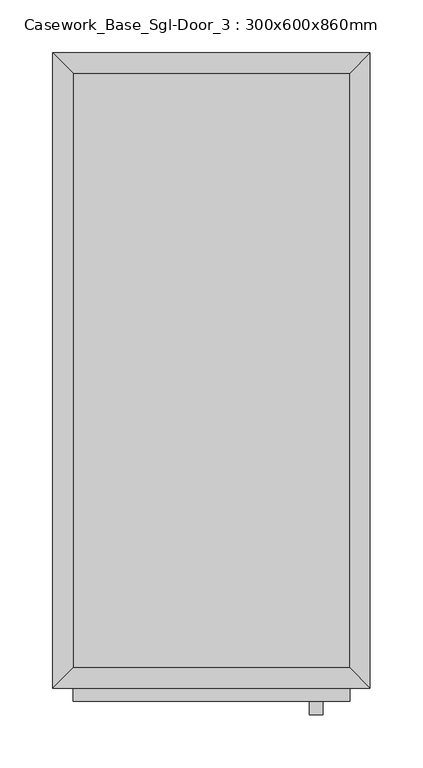
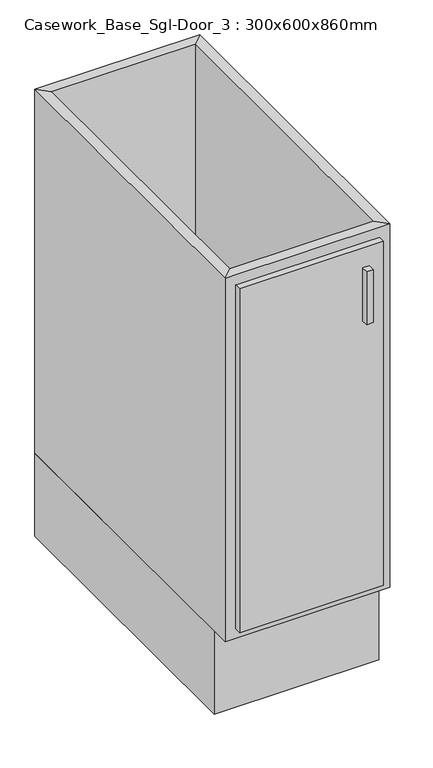
"""IFC4 building model written with IfcOpenShell, lengths in millimetres: furniture geometry, Casework_Base_Sgl-Door_3 : 300x600x860mm."""

from ifc_helpers import new_model, si_unit, frame, origin, origin_with_axes, place, context, project, spatial, polyline, outline, extrude, faceted_brep, source, transform, mapped, element, save


def casework_base_sgl_door_3_300x600x860mm_ce4f0042(model_context):
    return source(origin(), model_context, "Body", "SolidModel", [
        extrude(outline(polyline([(149.6877049, -19.05), (149.6877049, -580.95), (-112.2122951, -580.95), (-112.2122951, -19.05), (149.6877049, -19.05)])), frame((0.0, 0.0, 160.0), z_axis=(0.0, 0.0, 1.0), x_axis=(1.0, 0.0, 0.0)), (0.0, 0.0, 1.0), 19.05),
        faceted_brep([(149.6877049, -580.95, 860.0), (149.6877049, -580.95, 160.0), (-112.2122951, -580.95, 160.0), (-112.2122951, -580.95, 860.0), (168.7377049, -600.0, 860.0), (-131.2622951, -600.0, 860.0), (168.7377049, -600.0, 160.0), (-131.2622951, -600.0, 160.0), (-112.2122951, -19.05, 160.0), (-112.2122951, -19.05, 860.0), (-131.2622951, 0.0, 860.0), (-131.2622951, 0.0, 160.0), (149.6877049, -19.05, 160.0), (149.6877049, -19.05, 860.0), (168.7377049, 0.0, 860.0), (168.7377049, 0.0, 160.0)], [[[0, 1, 2, 3]], [[4, 0, 3, 5]], [[6, 4, 5, 7]], [[1, 6, 7, 2]], [[3, 2, 8, 9]], [[5, 3, 9, 10]], [[7, 5, 10, 11]], [[2, 7, 11, 8]], [[9, 8, 12, 13]], [[10, 9, 13, 14]], [[11, 10, 14, 15]], [[8, 11, 15, 12]], [[13, 12, 1, 0]], [[14, 13, 0, 4]], [[15, 14, 4, 6]], [[12, 15, 6, 1]]]),
        extrude(outline(polyline([(168.7377049, 0.0), (168.7377049, -565.0), (-131.2622951, -565.0), (-131.2622951, 0.0), (168.7377049, 0.0)])), origin_with_axes(), (0.0, 0.0, 1.0), 160.0),
        extrude(outline(polyline([(124.2877049, -625.4), (111.5877049, -625.4), (111.5877049, -612.7), (124.2877049, -612.7), (124.2877049, -625.4)])), frame((0.0, 0.0, 701.25), z_axis=(0.0, 0.0, 1.0), x_axis=(1.0, 0.0, 0.0)), (0.0, 0.0, 1.0), 101.6),
        extrude(outline(polyline([(149.6877049, -612.7), (-112.2122951, -612.7), (-112.2122951, -600.0), (149.6877049, -600.0), (149.6877049, -612.7)])), frame((0.0, 0.0, 179.05), z_axis=(0.0, 0.0, 1.0), x_axis=(1.0, 0.0, 0.0)), (0.0, 0.0, 1.0), 661.9),
    ])


if __name__ == "__main__":
    model = new_model("IFC4")
    model_context = context("Model", 3, world=origin())
    ifc_project = project(units=[si_unit("LENGTHUNIT", "METRE", prefix="MILLI")], contexts=[model_context])
    site = spatial("IfcSite", under=ifc_project)
    building = spatial("IfcBuilding", under=site)
    placement = place(None, origin())
    casework_base_sgl_door_3_300x600x860mm_shape = casework_base_sgl_door_3_300x600x860mm_ce4f0042(model_context)
    element("IfcFurniture", 1, ObjectType="Casework_Base_Sgl-Door_3 : 300x600x860mm", at=placement, inside=building, context=model_context, shape_type="MappedRepresentation", body=[
        mapped(casework_base_sgl_door_3_300x600x860mm_shape, transform((0.0, 0.0, 0.0), x_axis=(1.0, 0.0, 0.0), y_axis=(0.0, 1.0, 0.0), z_axis=(0.0, 0.0, 1.0))),
    ])
    save(model, "model.ifc")

# Revit data of these elements
# Type "Casework_Base_Sgl-Door_3 : 300x600x860mm"
#   Keynote = "N10"
#   Depth = 600 mm
#   Height = 860 mm
#   Plinth Depth = 35 mm
#   Plinth Height = 160 mm
#   Width = 300 mm
#   Material Cabinet = Cabinets
#   Material Door/Drawer = Cabinets
#   Material Handle = Cabinets - Handles
# Element 1 (IfcFurniture, "Casework_Base_Sgl-Door_3 : 300x600x860mm")
#   Materials on its faces: "Cabinets", "Cabinets - Handles"
# Materials
#   "Cabinets": class "Miscellaneous", colour RGB 249 249 249, transparency 0
#   "Cabinets - Handles": class "Metal", colour RGB 57 57 57, transparency 0
